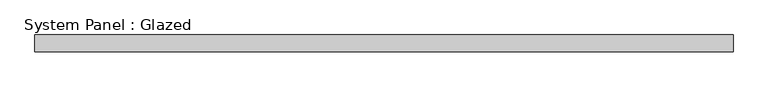
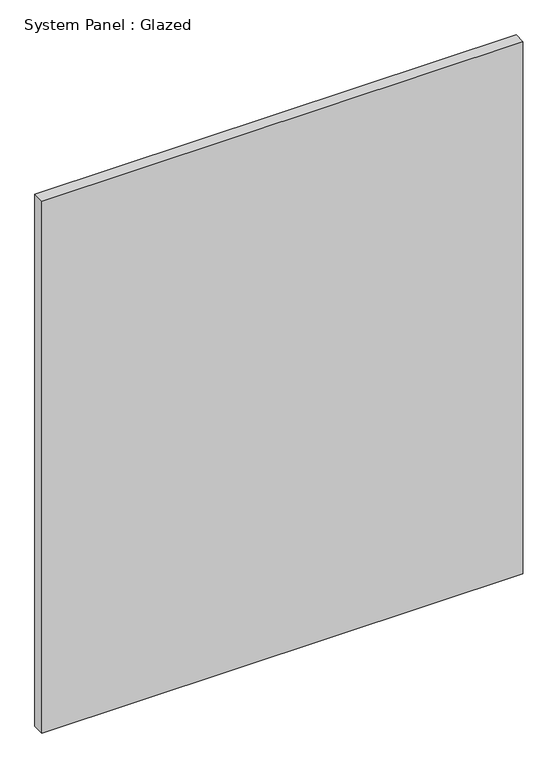
"""IFC4 building model written with IfcOpenShell, lengths in millimetres: plate geometry, System Panel : Glazed."""

from ifc_helpers import new_model, si_unit, origin, origin_with_axes, place, context, project, spatial, polyline, outline, extrude, source, transform, mapped, element, save


def system_panel_glazed_328a8357(model_context):
    return source(origin(), model_context, "Body", "SweptSolid", [
        extrude(outline(polyline([(521.5143964, 19.05), (-521.5143964, 19.05), (-521.5143964, 44.45), (521.5143964, 44.45), (521.5143964, 19.05)])), origin_with_axes(), (0.0, 0.0, 1.0), 1219.2),
    ])


if __name__ == "__main__":
    model = new_model("IFC4")
    model_context = context("Model", 3, world=origin())
    ifc_project = project(units=[si_unit("LENGTHUNIT", "METRE", prefix="MILLI")], contexts=[model_context])
    site = spatial("IfcSite", under=ifc_project)
    building = spatial("IfcBuilding", under=site)
    placement = place(None, origin())
    system_panel_glazed_shape = system_panel_glazed_328a8357(model_context)
    element("IfcPlate", 1, ObjectType="System Panel : Glazed", at=placement, inside=building, context=model_context, shape_type="MappedRepresentation", body=[
        mapped(system_panel_glazed_shape, transform((0.0, 0.0, 0.0), x_axis=(1.0, 0.0, 0.0), y_axis=(0.0, 1.0, 0.0), z_axis=(0.0, 0.0, 1.0))),
    ])
    save(model, "model.ifc")

# Revit data of these elements
# Element 1 (IfcPlate, "System Panel : Glazed")
#   Materials on its faces: "Glass"
# Materials
#   "Glass": class "Glass", colour RGB 0 128 192, transparency 0.75
